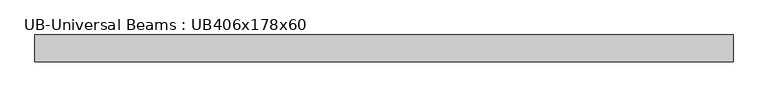
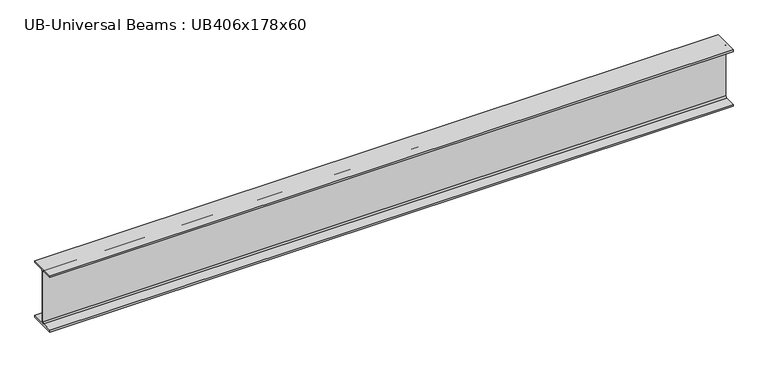
"""IFC4 building model written with IfcOpenShell, lengths in millimetres: beam geometry, UB-Universal Beams : UB406x178x60."""

from ifc_helpers import new_model, si_unit, point, frame, frame_2d, origin, place, context, project, spatial, polyline, circle_curve, trimmed, segment, composite_curve, outline, extrude, source, transform, mapped, element, save


def ub_universal_beams_ub406x178x60_0ea3e6ef(model_context):
    return source(origin(), model_context, "Body", "SweptSolid", [
        extrude(outline(composite_curve([segment(polyline([(88.95, -190.4), (88.95, -203.2), (-88.95, -203.2), (-88.95, -190.4), (-14.15, -190.4)]), True, "CONTINUOUS"), segment(trimmed(circle_curve(frame_2d((-14.15, -180.2)), 10.2), [point((-14.15, -190.4))], [point((-3.95, -180.2))], True, "CARTESIAN"), True, "CONTINUOUS"), segment(polyline([(-3.95, -180.2), (-3.95, 180.2)]), True, "CONTINUOUS"), segment(trimmed(circle_curve(frame_2d((-14.15, 180.2)), 10.2), [point((-3.95, 180.2))], [point((-14.15, 190.4))], True, "CARTESIAN"), True, "CONTINUOUS"), segment(polyline([(-14.15, 190.4), (-88.95, 190.4), (-88.95, 203.2), (88.95, 203.2), (88.95, 190.4), (14.15, 190.4)]), True, "CONTINUOUS"), segment(trimmed(circle_curve(frame_2d((14.15, 180.2)), 10.2), [point((14.15, 190.4))], [point((3.95, 180.2))], True, "CARTESIAN"), True, "CONTINUOUS"), segment(polyline([(3.95, 180.2), (3.95, -180.2)]), True, "CONTINUOUS"), segment(trimmed(circle_curve(frame_2d((14.15, -180.2)), 10.2), [point((3.95, -180.2))], [point((14.15, -190.4))], True, "CARTESIAN"), True, "CONTINUOUS"), segment(polyline([(14.15, -190.4), (88.95, -190.4)]), True, "CONTINUOUS")], self_intersect=False)), frame((-2301.35, 0.0, 0.0), z_axis=(1.0, 0.0, 0.0), x_axis=(0.0, 1.0, 0.0)), (0.0, 0.0, 1.0), 4653.7),
    ])


if __name__ == "__main__":
    model = new_model("IFC4")
    model_context = context("Model", 3, world=origin())
    ifc_project = project(units=[si_unit("LENGTHUNIT", "METRE", prefix="MILLI")], contexts=[model_context])
    site = spatial("IfcSite", under=ifc_project)
    building = spatial("IfcBuilding", under=site)
    placement = place(None, origin())
    ub_universal_beams_ub406x178x60_shape = ub_universal_beams_ub406x178x60_0ea3e6ef(model_context)
    element("IfcBeam", 1, ObjectType="UB-Universal Beams : UB406x178x60", at=placement, inside=building, context=model_context, shape_type="MappedRepresentation", body=[
        mapped(ub_universal_beams_ub406x178x60_shape, transform((0.0, 0.0, 0.0), x_axis=(1.0, 0.0, 0.0), y_axis=(0.0, 1.0, 0.0), z_axis=(0.0, 0.0, 1.0))),
    ])
    save(model, "model.ifc")

# Revit data of these elements
# Type "UB-Universal Beams : UB406x178x60"
#   Section Name Key = "UB406X178X60"
#   Width = 17.79 cm
#   Web Thickness = 0.79 cm
#   Web Fillet = 1.02 cm
#   Warping Constant = 466000.0 cm⁶
#   Torsional Moment of Inertia = 33.30 cm⁴
#   Section Area = 76.5 cm²
#   Plastic Modulus weak axis = 209.0 cm³
#   Plastic Modulus strong axis = 1200.0 cm³
#   Nominal Weight = 60.0998 kgf/m
#   Moment of Inertia weak axis = 1203.00 cm⁴
#   Moment of Inertia strong axis = 21596.00 cm⁴
#   Height = 40.64 cm
#   Flange Thickness = 1.28 cm
#   Elastic Modulus weak axis = 135.0 cm³
#   Elastic Modulus strong axis = 1063.0 cm³
#   Centroid Vertical = 20.32 cm
#   Centroid Horizontal = 8.895 cm
#   Bolt Spacing = 9.0 cm
#   Length [instance default] = 1500 mm
#   Structural Material [instance default] = Metal - Steel 43-275
#   Type Comments = ""
#   Assembly Code = ""
# Element 1 (IfcBeam, "UB-Universal Beams : UB406x178x60")
#   Materials on its faces: "Metal - Steel 43-275"
# Materials
#   "Metal - Steel 43-275": class "Metal", colour RGB 247 247 247, transparency 0, Cost = 0
